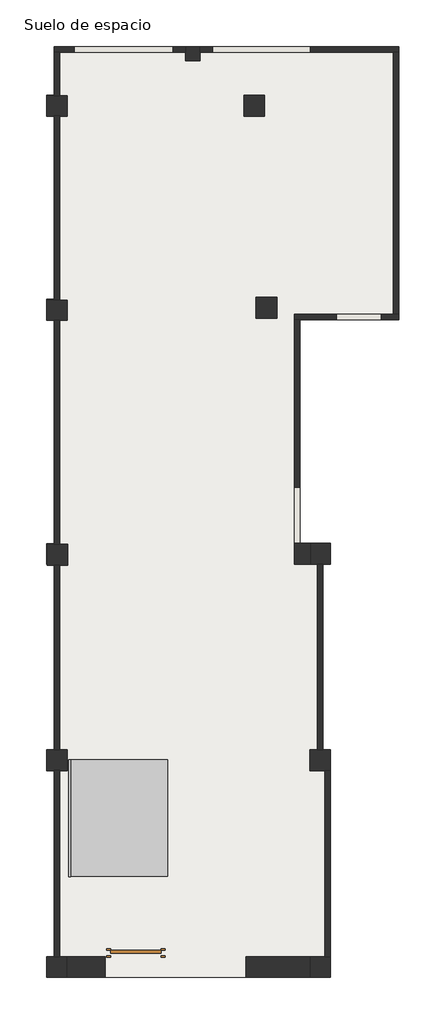
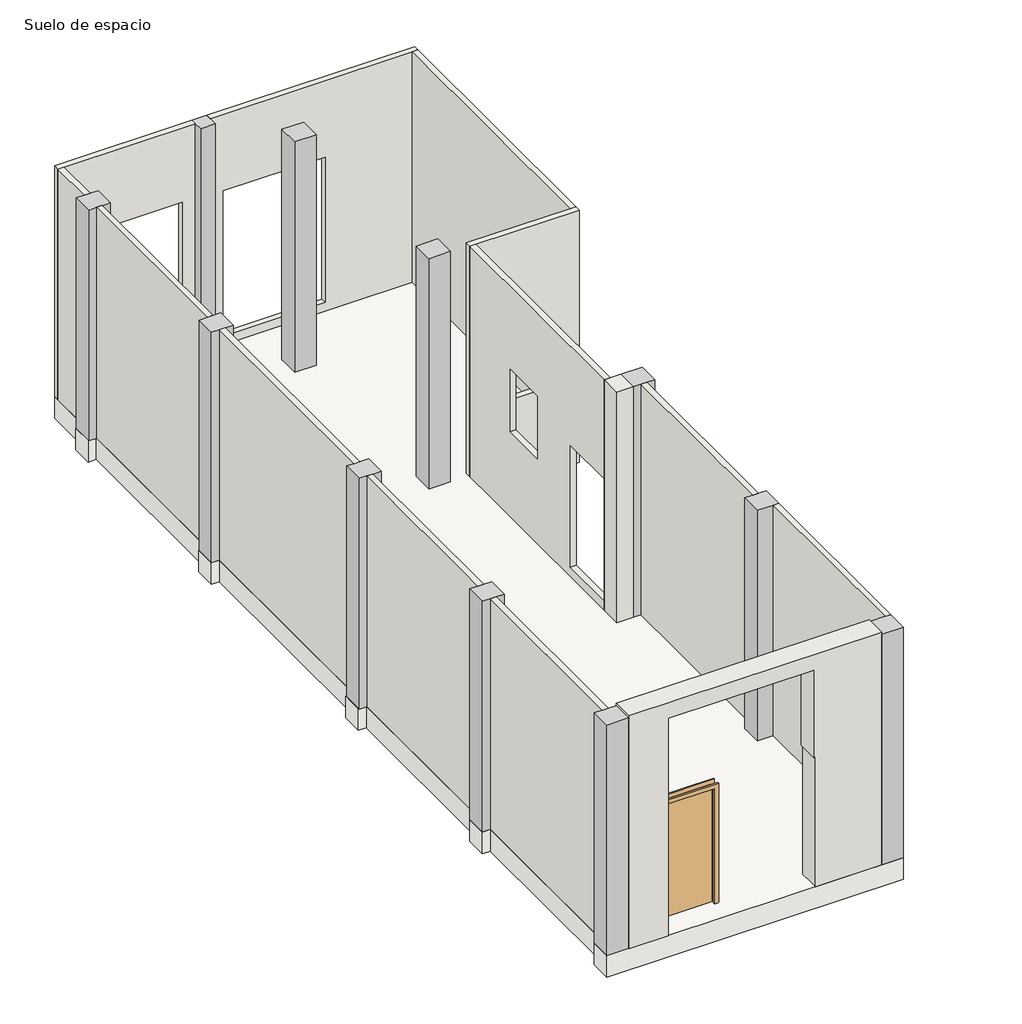
# One storey: 14 walls, 11 columns, 1 door, 1 railing, 1 ramp, 1 slab.
"""IFC4 building model written with IfcOpenShell, lengths in millimetres."""

import ifcopenshell
import ifcopenshell.guid

model = None  # the IFC model being written
_history = None  # IfcOwnerHistory: only IFC2X3 demands one
_inside = {}  # id of a spatial element -> (the spatial element, [elements in it])
_under = {}  # id of a project, library or spatial element -> (it, [spatial elements below it])
_declared = {}  # id of a project -> (the project, [libraries it declares])
_typed = {}  # id of a type object -> (the type object, [elements of that type])
_made_of = {}  # id of a material, layer set ... -> (it, [elements and type objects made of it])


def new_model(schema):
    """Start an empty IFC model of exactly this schema.

    Asked for "IFC4X3", IfcOpenShell would pick the latest addendum, in which some entities
    have other attributes; the version numbers below select the first issue.
    IFC2X3 requires an IfcOwnerHistory on every rooted entity: one is made here for all.
    """
    global model, _history
    if schema == "IFC4X3":
        model = ifcopenshell.file(schema_version=(4, 3, 0, 0))
    else:
        model = ifcopenshell.file(schema=schema)
    _inside.clear()
    _under.clear()
    _declared.clear()
    _typed.clear()
    _made_of.clear()
    _history = None
    if model.schema == "IFC2X3":
        org = make("IfcOrganization", Name="unknown")
        user = make(
            "IfcPersonAndOrganization",
            ThePerson=make("IfcPerson", FamilyName="unknown"),
            TheOrganization=org,
        )
        app = make(
            "IfcApplication",
            ApplicationDeveloper=org,
            Version="unknown",
            ApplicationFullName="unknown",
            ApplicationIdentifier="unknown",
        )
        _history = make(
            "IfcOwnerHistory",
            OwningUser=user,
            OwningApplication=app,
            ChangeAction="ADDED",
            CreationDate=0,
        )
    return model


def make(cls, **values):
    """One entity of the class cls with the attributes given. An attribute that is None is left unset."""
    return model.create_entity(
        cls, **{name: value for name, value in values.items() if value is not None}
    )


def rooted(cls, **values):
    """An entity with a GlobalId (a new one), such as an element, a storey or a relation."""
    return make(cls, GlobalId=ifcopenshell.guid.new(), OwnerHistory=_history, **values)


def si_unit(unit_type, name, prefix=None):
    """IfcSIUnit, for example si_unit("LENGTHUNIT", "METRE", prefix="MILLI")."""
    return make("IfcSIUnit", UnitType=unit_type, Prefix=prefix, Name=name)


def assignment(units):
    """IfcUnitAssignment: the units of a project."""
    return None if units is None else make("IfcUnitAssignment", Units=units)


def point(xyz):
    """IfcCartesianPoint."""
    return None if xyz is None else make("IfcCartesianPoint", Coordinates=xyz)


def direction(xyz):
    """IfcDirection."""
    return None if xyz is None else make("IfcDirection", DirectionRatios=xyz)


def frame(location, z_axis=None, x_axis=None):
    """IfcAxis2Placement3D, a coordinate frame: its origin and axes. An axis left out is left unset."""
    return make(
        "IfcAxis2Placement3D",
        Location=point(location),
        Axis=direction(z_axis),
        RefDirection=direction(x_axis),
    )


def origin():
    """The frame at (0, 0, 0) with its axes left unset."""
    return frame((0.0, 0.0, 0.0))


def origin_with_axes():
    """The frame at (0, 0, 0) with the z axis (0, 0, 1) and the x axis (1, 0, 0) written out."""
    return frame((0.0, 0.0, 0.0), z_axis=(0.0, 0.0, 1.0), x_axis=(1.0, 0.0, 0.0))


def place(relative_to, where):
    """IfcLocalPlacement: puts the frame where relative to a parent placement (None: the world)."""
    return make(
        "IfcLocalPlacement", PlacementRelTo=relative_to, RelativePlacement=where
    )


def context(
    kind, dimensions, precision=None, world=None, true_north=None, identifier=None
):
    """IfcGeometricRepresentationContext, for example the 3D "Model" context."""
    return make(
        "IfcGeometricRepresentationContext",
        ContextIdentifier=identifier,
        ContextType=kind,
        CoordinateSpaceDimension=dimensions,
        Precision=precision,
        WorldCoordinateSystem=world,
        TrueNorth=true_north,
    )


def project(units=None, contexts=None):
    """IfcProject with its units and contexts."""
    return rooted(
        "IfcProject",
        Name="project",
        RepresentationContexts=contexts,
        UnitsInContext=assignment(units),
    )


def spatial(cls, under=None, at=None, **own):
    """A site, building, storey or space (cls), placed at a placement, below another one or the project."""
    s = rooted(cls, ObjectPlacement=at, **own)
    if under is not None:
        _under.setdefault(under.id(), (under, []))[1].append(s)
    return s


def polyline(points):
    """IfcPolyline through the points."""
    return make("IfcPolyline", Points=[point(p) for p in points])


def ellipse_curve(where, semi_axis1, semi_axis2):
    """IfcEllipse in the frame where."""
    return make(
        "IfcEllipse", Position=where, SemiAxis1=semi_axis1, SemiAxis2=semi_axis2
    )


def outline(outer, holes=None, kind="AREA"):
    """IfcArbitraryClosedProfileDef: a profile drawn as a closed curve; with holes, ...WithVoids."""
    if holes is None:
        return make("IfcArbitraryClosedProfileDef", ProfileType=kind, OuterCurve=outer)
    return make(
        "IfcArbitraryProfileDefWithVoids",
        ProfileType=kind,
        OuterCurve=outer,
        InnerCurves=holes,
    )


def extrude(swept, where, along, depth):
    """IfcExtrudedAreaSolid: the profile swept, set in the frame where, extruded along a direction by depth."""
    return make(
        "IfcExtrudedAreaSolid",
        SweptArea=swept,
        Position=where,
        ExtrudedDirection=direction(along),
        Depth=depth,
    )


def faces_of(points, faces, orient=None, outer=None):
    """IfcFace entities. A face is a list of loops; a loop is a list of indices into points, from 0.

    orient and outer hold one flag for each loop. By default every Orientation is true, the
    first loop of a face is its IfcFaceOuterBound and the others are IfcFaceBound.
    """
    made = []
    for i, loops in enumerate(faces):
        bounds = []
        for j, loop in enumerate(loops):
            is_outer = j == 0 if outer is None else outer[i][j]
            bounds.append(
                make(
                    "IfcFaceOuterBound" if is_outer else "IfcFaceBound",
                    Bound=make("IfcPolyLoop", Polygon=[points[k] for k in loop]),
                    Orientation=True if orient is None else orient[i][j],
                )
            )
        made.append(make("IfcFace", Bounds=bounds))
    return made


def faceted_brep(points, faces, orient=None, outer=None, voids=None):
    """IfcFacetedBrep: a solid bounded by flat faces; with voids (closed shells), ...WithVoids."""
    shared = [point(p) for p in points]
    hull = make("IfcClosedShell", CfsFaces=faces_of(shared, faces, orient, outer))
    if voids is None:
        return make("IfcFacetedBrep", Outer=hull)
    return make(
        "IfcFacetedBrepWithVoids",
        Outer=hull,
        Voids=[
            make(cls, CfsFaces=faces_of(shared, fs, o, b)) for cls, fs, o, b in voids
        ],
    )


def shape(context_of_items, identifier, shape_type, items):
    """IfcShapeRepresentation: the items that make up one representation, for example the "Body"."""
    return make(
        "IfcShapeRepresentation",
        ContextOfItems=context_of_items,
        RepresentationIdentifier=identifier,
        RepresentationType=shape_type,
        Items=items,
    )


def source(mapping_origin, context_of_items, identifier, shape_type, items):
    """IfcRepresentationMap: a shape defined once, which mapped items show again and again."""
    return make(
        "IfcRepresentationMap",
        MappingOrigin=mapping_origin,
        MappedRepresentation=shape(context_of_items, identifier, shape_type, items),
    )


def transform(
    local_origin,
    x_axis=None,
    y_axis=None,
    z_axis=None,
    scale=None,
    scale2=None,
    scale3=None,
    uniform=True,
):
    """IfcCartesianTransformationOperator3D, or its non-uniform kind. x_axis, y_axis, z_axis: its Axis1, 2, 3."""
    if uniform:
        return make(
            "IfcCartesianTransformationOperator3D",
            Axis1=direction(x_axis),
            Axis2=direction(y_axis),
            LocalOrigin=point(local_origin),
            Scale=scale,
            Axis3=direction(z_axis),
        )
    return make(
        "IfcCartesianTransformationOperator3DnonUniform",
        Axis1=direction(x_axis),
        Axis2=direction(y_axis),
        LocalOrigin=point(local_origin),
        Scale=scale,
        Axis3=direction(z_axis),
        Scale2=scale2,
        Scale3=scale3,
    )


def mapped(mapping_source, mapping_target):
    """IfcMappedItem: shows the shape of a source again, moved by a transform."""
    return make(
        "IfcMappedItem", MappingSource=mapping_source, MappingTarget=mapping_target
    )


def made_of(thing, what):
    """Note that an element or type object is made of a material, layer set ...; save() writes the relation."""
    if what is not None:
        _made_of.setdefault(what.id(), (what, []))[1].append(thing)
    return thing


def element(
    cls,
    number,
    at=None,
    inside=None,
    cuts=None,
    type_object=None,
    material=None,
    context=None,
    identifier="Body",
    shape_type=None,
    held_by="IfcProductDefinitionShape",
    body=None,
    shapes=None,
    **own,
):
    """One element of the class cls, such as IfcWall. Its Tag is "e" and its number.

    at: its placement. inside: the storey or other place that contains it. cuts: it is an
    opening in that element (IfcRelVoidsElement). A single representation is given by context,
    identifier, shape_type and body (its items); several are given by shapes. held_by: the class
    of the entity that holds the representations. save() writes the other relations.
    """
    e = rooted(cls, Tag="e%d" % number, ObjectPlacement=at, **own)
    if body is not None:
        shapes = [shape(context, identifier, shape_type, body)]
    if shapes is not None:
        e.Representation = make(held_by, Representations=shapes)
    if inside is not None:
        _inside.setdefault(inside.id(), (inside, []))[1].append(e)
    if cuts is not None:
        rooted(
            "IfcRelVoidsElement", RelatingBuildingElement=cuts, RelatedOpeningElement=e
        )
    if type_object is not None:
        _typed.setdefault(type_object.id(), (type_object, []))[1].append(e)
    return made_of(e, material)


def aggregate(whole, parts):
    """IfcRelAggregates: a whole, such as a stair, and the parts it consists of."""
    return rooted("IfcRelAggregates", RelatingObject=whole, RelatedObjects=parts)


def save(model, path):
    """Write the relations noted so far, then the file.

    IfcRelAggregates (storeys below a building ...), IfcRelContainedInSpatialStructure (elements
    in a storey), IfcRelDefinesByType, IfcRelAssociatesMaterial and IfcRelDeclares: one each for
    every whole, place, type object, material and project.
    """
    for whole, parts in _under.values():
        aggregate(whole, parts)
    for where, things in _inside.values():
        rooted(
            "IfcRelContainedInSpatialStructure",
            RelatedElements=things,
            RelatingStructure=where,
        )
    for kind, things in _typed.values():
        rooted("IfcRelDefinesByType", RelatedObjects=things, RelatingType=kind)
    for what, things in _made_of.values():
        rooted("IfcRelAssociatesMaterial", RelatedObjects=things, RelatingMaterial=what)
    for by, libraries in _declared.values():
        rooted("IfcRelDeclares", RelatingContext=by, RelatedDefinitions=libraries)
    model.write(path)


def plane_surface(at):
    """IfcPlane: the flat surface through the origin of the frame at, square to its z axis."""
    return make("IfcPlane", Position=at)


def cylinder_surface(at, radius):
    """IfcCylindricalSurface: all points at the distance radius from the z axis of the frame at."""
    return make("IfcCylindricalSurface", Position=at, Radius=radius)


def advanced_brep(points, edges, surfaces, faces):
    """IfcAdvancedBrep: a solid bounded by faces that lie on surfaces and meet in shared edges.

    An edge is (start, end): straight between two places in points (the first is 0);
    or (start, end, curve); or (start, end, curve, False) where it runs against its curve.
    A face is (place in surfaces, loops), or (place, loops, False) where it looks against
    its surface's normal. A loop lists edges by number (the first is 1), with a minus sign
    where the edge is run from its end to its start. The first loop is the outer one.
    """
    corners = [point(p) for p in points]
    vertices = [make("IfcVertexPoint", VertexGeometry=c) for c in corners]
    made = []
    for start, end, *more in edges:
        made.append(
            make(
                "IfcEdgeCurve",
                EdgeStart=vertices[start],
                EdgeEnd=vertices[end],
                EdgeGeometry=more[0] if more else make("IfcPolyline", Points=[corners[start], corners[end]]),
                SameSense=more[1] if len(more) > 1 else True,
            )
        )
    hull = []
    for where, loops, *sense in faces:
        bounds = []
        for j, loop in enumerate(loops):
            ring = [make("IfcOrientedEdge", EdgeElement=made[abs(k) - 1], Orientation=k > 0) for k in loop]
            bounds.append(
                make(
                    "IfcFaceOuterBound" if j == 0 else "IfcFaceBound",
                    Bound=make("IfcEdgeLoop", EdgeList=ring),
                    Orientation=True,
                )
            )
        hull.append(make("IfcAdvancedFace", Bounds=bounds, FaceSurface=surfaces[where], SameSense=sense[0] if sense else True))
    return make("IfcAdvancedBrep", Outer=make("IfcClosedShell", CfsFaces=hull))


def m_rectangular_column_380_x_380mm_f7aa0fc7(model_context):
    return source(origin(), model_context, "Body", "SweptSolid", [
        extrude(outline(polyline([(190.0, 190.0), (190.0, -190.0), (-190.0, -190.0), (-190.0, 190.0), (190.0, 190.0)])), frame((0.0, 0.0, 40.0), z_axis=(0.0, 0.0, 1.0), x_axis=(1.0, 0.0, 0.0)), (0.0, 0.0, 1.0), 4260.0),
    ])


def m_single_flush_0915_x_2134mm_17617764(model_context):
    return source(origin(), model_context, "Body", "SweptSolid", [
        extrude(outline(polyline([(2210.0, -533.5), (0.0, -533.5), (0.0, -457.5), (2134.0, -457.5), (2134.0, 457.5), (0.0, 457.5), (0.0, 533.5), (2210.0, 533.5), (2210.0, -533.5)])), frame((0.0, -75.0, 0.0), z_axis=(0.0, 1.0, 0.0), x_axis=(0.0, 0.0, 1.0)), (0.0, 0.0, 1.0), 25.0),
        extrude(outline(polyline([(2210.0, 533.5), (2210.0, -533.5), (0.0, -533.5), (0.0, -457.5), (2134.0, -457.5), (2134.0, 457.5), (0.0, 457.5), (0.0, 533.5), (2210.0, 533.5)])), frame((0.0, 50.0, 0.0), z_axis=(0.0, 1.0, 0.0), x_axis=(0.0, 0.0, 1.0)), (0.0, 0.0, 1.0), 25.0),
        extrude(outline(polyline([(457.5, 1.0), (457.5, -50.0), (-457.5, -50.0), (-457.5, 1.0), (457.5, 1.0)])), origin_with_axes(), (0.0, 0.0, 1.0), 2134.0),
    ])


def ramp_1_66d68c1d(model_context):
    return source(origin(), model_context, "Body", "SweptSolid", [
        extrude(outline(polyline([(-178.9025016, 40.0), (1960.7723822, 200.0), (1960.7723822, 49.5812066), (-178.9025016, -110.4187934), (-178.9025016, 40.0)])), frame((5764.7203549, 0.0, 0.0), z_axis=(1.0, 0.0, 0.0), x_axis=(0.0, 1.0, 0.0)), (0.0, 0.0, 1.0), 1790.0),
    ])


model = new_model("IFC4")

# Units and contexts
model_context = context("Model", 3, world=origin())
ifc_project = project(units=[si_unit("LENGTHUNIT", "METRE", prefix="MILLI")], contexts=[model_context])

# Site, building, storey
site = spatial("IfcSite", under=ifc_project)
building = spatial("IfcBuilding", under=site)
storey = spatial("IfcBuildingStorey", under=building, Name="Suelo de espacio", Elevation=40.0)

# Columns
placement = place(None, origin())
element("IfcColumn", 1, ObjectType="M_Rectangular Column : 260 x 260mm", at=placement, inside=storey, context=model_context, shape_type="Brep", body=[
    faceted_brep([(8142.3508412, 14950.939444, 4300.0), (7882.3508412, 14950.939444, 4300.0), (7882.3508412, 14850.939444, 4300.0), (7882.3508412, 14690.939444, 4300.0), (8142.3508412, 14690.939444, 4300.0), (8142.3508412, 14850.939444, 4300.0), (8142.3508412, 14950.939444, 40.0), (8142.3508412, 14850.939444, 40.0), (8142.3508412, 14690.939444, 40.0), (7882.3508412, 14690.939444, 40.0), (7882.3508412, 14850.939444, 40.0), (7882.3508412, 14950.939444, 40.0)], [[[0, 1, 2, 3, 4, 5]], [[6, 7, 8, 9, 10, 11]], [[1, 0, 6, 11]], [[3, 2, 1, 11, 10, 9]], [[4, 3, 9, 8]], [[0, 5, 4, 8, 7, 6]]]),
])
element("IfcColumn", 2, ObjectType="M_Rectangular Column : 380 x 370mm", at=placement, inside=storey, context=model_context, shape_type="Brep", body=[
    faceted_brep([(5722.3508412, 10330.939444, 4300.0), (5342.3508412, 10330.939444, 4300.0), (5342.3508412, 9960.939444, 4300.0), (5482.3508412, 9960.939444, 4300.0), (5582.3508412, 9960.939444, 4300.0), (5722.3508412, 9960.939444, 4300.0), (5722.3508412, 10330.939444, 40.0), (5722.3508412, 9960.939444, 40.0), (5582.3508412, 9960.939444, 40.0), (5482.3508412, 9960.939444, 40.0), (5342.3508412, 9960.939444, 40.0), (5342.3508412, 10330.939444, 40.0)], [[[0, 1, 2, 3, 4, 5]], [[6, 7, 8, 9, 10, 11]], [[1, 0, 6, 11]], [[2, 1, 11, 10]], [[5, 4, 3, 2, 10, 9, 8, 7]], [[0, 5, 7, 6]]]),
])
element("IfcColumn", 3, ObjectType="M_Rectangular Column : 380 x 370mm", at=placement, inside=storey, context=model_context, shape_type="Brep", body=[
    faceted_brep([(5722.3508412, 14050.939444, 4300.0), (5582.3508412, 14050.939444, 4300.0), (5482.3508412, 14050.939444, 4300.0), (5342.3508412, 14050.939444, 4300.0), (5342.3508412, 13680.939444, 4300.0), (5482.3508412, 13680.939444, 4300.0), (5482.3508412, 13685.939444, 4300.0), (5582.3508412, 13685.939444, 4300.0), (5582.3508412, 13680.939444, 4300.0), (5722.3508412, 13680.939444, 4300.0), (5722.3508412, 14050.939444, 40.0), (5722.3508412, 13680.939444, 40.0), (5582.3508412, 13680.939444, 40.0), (5582.3508412, 13685.939444, 40.0), (5482.3508412, 13685.939444, 40.0), (5482.3508412, 13680.939444, 40.0), (5342.3508412, 13680.939444, 40.0), (5342.3508412, 14050.939444, 40.0), (5482.3508412, 14050.939444, 40.0), (5582.3508412, 14050.939444, 40.0)], [[[0, 1, 2, 3, 4, 5, 6, 7, 8, 9]], [[10, 11, 12, 13, 14, 15, 16, 17, 18, 19]], [[3, 2, 1, 0, 10, 19, 18, 17]], [[4, 3, 17, 16]], [[4, 16, 15, 5]], [[0, 9, 11, 10]], [[7, 13, 12, 8]], [[14, 6, 5, 15]], [[13, 7, 6, 14]], [[11, 9, 8, 12]]]),
])
element("IfcColumn", 4, ObjectType="M_Rectangular Column : 380 x 380mm", at=placement, inside=storey, context=model_context, shape_type="Brep", body=[
    faceted_brep([(5722.3508412, -1629.060556, 4300.0), (5582.3508412, -1629.060556, 4300.0), (5482.3508412, -1629.060556, 4300.0), (5342.3508412, -1629.060556, 4300.0), (5342.3508412, -2009.060556, 4300.0), (5722.3508412, -2009.060556, 4300.0), (5722.3508412, -1629.060556, 40.0), (5722.3508412, -2009.060556, 40.0), (5342.3508412, -2009.060556, 40.0), (5342.3508412, -1629.060556, 40.0), (5482.3508412, -1629.060556, 40.0), (5582.3508412, -1629.060556, 40.0)], [[[0, 1, 2, 3, 4, 5]], [[6, 7, 8, 9, 10, 11]], [[3, 2, 1, 0, 6, 11, 10, 9]], [[4, 3, 9, 8]], [[5, 4, 8, 7]], [[0, 5, 7, 6]]]),
])
element("IfcColumn", 5, ObjectType="M_Rectangular Column : 380 x 380mm", at=placement, inside=storey, context=model_context, shape_type="Brep", body=[
    faceted_brep([(10522.3508412, -1629.060556, 4300.0), (10422.3508412, -1629.060556, 4300.0), (10142.3508412, -1629.060556, 4300.0), (10142.3508412, -2009.060556, 4300.0), (10522.3508412, -2009.060556, 4300.0), (10522.3508412, -1629.060556, 40.0), (10522.3508412, -2009.060556, 40.0), (10142.3508412, -2009.060556, 40.0), (10142.3508412, -1629.060556, 40.0), (10422.3508412, -1629.060556, 40.0)], [[[0, 1, 2, 3, 4]], [[5, 6, 7, 8, 9]], [[2, 1, 0, 5, 9, 8]], [[3, 2, 8, 7]], [[4, 3, 7, 6]], [[0, 4, 6, 5]]]),
])
element("IfcColumn", 6, ObjectType="M_Rectangular Column : 380 x 380mm", at=placement, inside=storey, context=model_context, shape_type="Brep", body=[
    faceted_brep([(5722.3508412, 2140.939444, 4300.0), (5582.3508412, 2140.939444, 4300.0), (5482.3508412, 2140.939444, 4300.0), (5342.3508412, 2140.939444, 4300.0), (5342.3508412, 1760.939444, 4300.0), (5482.3508412, 1760.939444, 4300.0), (5482.3508412, 1761.3849652, 4300.0), (5582.3508412, 1761.3849652, 4300.0), (5582.3508412, 1760.939444, 4300.0), (5722.3508412, 1760.939444, 4300.0), (5722.3508412, 2140.939444, 40.0), (5722.3508412, 1760.939444, 40.0), (5582.3508412, 1760.939444, 40.0), (5582.3508412, 1761.3849652, 40.0), (5482.3508412, 1761.3849652, 40.0), (5482.3508412, 1760.939444, 40.0), (5342.3508412, 1760.939444, 40.0), (5342.3508412, 2140.939444, 40.0), (5482.3508412, 2140.939444, 40.0), (5582.3508412, 2140.939444, 40.0)], [[[0, 1, 2, 3, 4, 5, 6, 7, 8, 9]], [[10, 11, 12, 13, 14, 15, 16, 17, 18, 19]], [[3, 2, 1, 0, 10, 19, 18, 17]], [[4, 3, 17, 16]], [[4, 16, 15, 5]], [[0, 9, 11, 10]], [[7, 13, 12, 8]], [[14, 6, 5, 15]], [[11, 9, 8, 12]], [[13, 7, 6, 14]]]),
])
element("IfcColumn", 7, ObjectType="M_Rectangular Column : 380 x 380mm", at=placement, inside=storey, context=model_context, shape_type="Brep", body=[
    faceted_brep([(10522.3508412, 2140.939444, 4300.0), (10382.3508412, 2140.939444, 4300.0), (10282.3508412, 2140.939444, 4300.0), (10142.3508412, 2140.939444, 4300.0), (10142.3508412, 1760.939444, 4300.0), (10422.3508412, 1760.939444, 4300.0), (10522.3508412, 1760.939444, 4300.0), (10522.3508412, 2140.939444, 40.0), (10522.3508412, 1760.939444, 40.0), (10422.3508412, 1760.939444, 40.0), (10142.3508412, 1760.939444, 40.0), (10142.3508412, 2140.939444, 40.0), (10282.3508412, 2140.939444, 40.0), (10382.3508412, 2140.939444, 40.0)], [[[0, 1, 2, 3, 4, 5, 6]], [[7, 8, 9, 10, 11, 12, 13]], [[3, 2, 1, 0, 7, 13, 12, 11]], [[4, 3, 11, 10]], [[6, 5, 4, 10, 9, 8]], [[0, 6, 8, 7]]]),
])
element("IfcColumn", 8, ObjectType="M_Rectangular Column : 380 x 380mm", at=placement, inside=storey, context=model_context, shape_type="Brep", body=[
    faceted_brep([(5732.3508412, 5880.939444, 4300.0), (5582.3508412, 5880.939444, 4300.0), (5482.3508412, 5880.939444, 4300.0), (5352.3508412, 5880.939444, 4300.0), (5352.3508412, 5500.939444, 4300.0), (5482.3508412, 5500.939444, 4300.0), (5582.3508412, 5500.939444, 4300.0), (5732.3508412, 5500.939444, 4300.0), (5732.3508412, 5880.939444, 40.0), (5732.3508412, 5500.939444, 40.0), (5582.3508412, 5500.939444, 40.0), (5482.3508412, 5500.939444, 40.0), (5352.3508412, 5500.939444, 40.0), (5352.3508412, 5880.939444, 40.0), (5482.3508412, 5880.939444, 40.0), (5582.3508412, 5880.939444, 40.0)], [[[0, 1, 2, 3, 4, 5, 6, 7]], [[8, 9, 10, 11, 12, 13, 14, 15]], [[3, 2, 1, 0, 8, 15, 14, 13]], [[4, 3, 13, 12]], [[7, 6, 5, 4, 12, 11, 10, 9]], [[0, 7, 9, 8]]]),
])
element("IfcColumn", 9, ObjectType="M_Rectangular Column : 380 x 380mm", at=placement, inside=storey, context=model_context, shape_type="Brep", body=[
    faceted_brep([(10522.3508412, 5520.939444, 4300.0), (10522.3508412, 5900.939444, 4300.0), (10152.3508412, 5900.939444, 4300.0), (10152.3508412, 5520.939444, 4300.0), (10282.3508412, 5520.939444, 4300.0), (10382.3508412, 5520.939444, 4300.0), (10522.3508412, 5900.939444, 40.0), (10522.3508412, 5520.939444, 40.0), (10382.3508412, 5520.939444, 40.0), (10282.3508412, 5520.939444, 40.0), (10152.3508412, 5520.939444, 40.0), (10152.3508412, 5900.939444, 40.0)], [[[0, 1, 2, 3, 4, 5]], [[6, 7, 8, 9, 10, 11]], [[1, 6, 11, 2]], [[7, 0, 5, 4, 3, 10, 9, 8]], [[1, 0, 7, 6]], [[3, 2, 11, 10]]]),
])
m_rectangular_column_380_x_380mm_shape = m_rectangular_column_380_x_380mm_f7aa0fc7(model_context)
element("IfcColumn", 10, ObjectType="M_Rectangular Column : 380 x 380mm", at=placement, inside=storey, context=model_context, shape_type="MappedRepresentation", body=[
    mapped(m_rectangular_column_380_x_380mm_shape, transform((9132.3508412, 13870.939444, 0.0), x_axis=(1.0, 0.0, 0.0), y_axis=(0.0, 1.0, 0.0), z_axis=(0.0, 0.0, 1.0))),
])
element("IfcColumn", 11, ObjectType="M_Rectangular Column : 380 x 380mm", at=placement, inside=storey, context=model_context, shape_type="MappedRepresentation", body=[
    mapped(m_rectangular_column_380_x_380mm_shape, transform((9352.3508412, 10190.939444, 0.0), x_axis=(1.0, 0.0, 0.0), y_axis=(0.0, 1.0, 0.0), z_axis=(0.0, 0.0, 1.0))),
])

# Door
m_single_flush_0915_x_2134mm_shape = m_single_flush_0915_x_2134mm_17617764(model_context)
element("IfcDoor", 12, ObjectType="M_Single-Flush : 0915 x 2134mm", at=placement, inside=storey, context=model_context, shape_type="MappedRepresentation", body=[
    mapped(m_single_flush_0915_x_2134mm_shape, transform((6972.3508412, -1564.060556, 40.0), x_axis=(-1.0, 0.0, 0.0), y_axis=(0.0, -1.0, 0.0), z_axis=(0.0, 0.0, 1.0))),
])

# Railing
element("IfcRailing", 13, ObjectType="900mm Pipe", at=placement, inside=storey, context=model_context, shape_type="AdvancedBrep", body=[
    advanced_brep(
    [(5784.7203549, -178.9025016, 919.9441609), (5744.7203549, -178.9025016, 919.9441609), (5784.7203549, 1960.7723822, 1079.9441609), (5744.7203549, 1960.7723822, 1079.9441609)],
    [
        (0, 1, ellipse_curve(frame((5764.7203549, -178.9025016, 919.9441609), z_axis=(0.0, -1.0, 0.0), x_axis=(0.0, 0.0, -0.9999999999999999)), 20.0558391, 20.0)),
        (1, 0, ellipse_curve(frame((5764.7203549, -178.9025016, 919.9441609), z_axis=(0.0, -1.0, 0.0), x_axis=(0.0, 0.0, -0.9999999999999999)), 20.0558391, 20.0)),
        (2, 3, ellipse_curve(frame((5764.7203549, 1960.7723822, 1079.9441609), z_axis=(0.0, 1.0, 0.0), x_axis=(0.0, 0.0, -0.9999999999999999)), 20.0558391, 20.0)),
        (3, 2, ellipse_curve(frame((5764.7203549, 1960.7723822, 1079.9441609), z_axis=(0.0, 1.0, 0.0), x_axis=(0.0, 0.0, -0.9999999999999999)), 20.0558391, 20.0)),
        (0, 2),
        (3, 1),
    ],
    [
        plane_surface(frame((5764.7203549, -178.9025016, 940.0), z_axis=(0.0, -1.0, 0.0), x_axis=(0.0, 0.0, 1.0))),
        plane_surface(frame((5764.7203549, 1960.7723822, 1100.0), z_axis=(0.0, 1.0, 0.0), x_axis=(0.0, 0.0, 1.0))),
        cylinder_surface(frame((5764.7203549, -177.4111112, 920.0556837), z_axis=(0.0, -0.9972158174462339, -0.07456952081809042), x_axis=(-1.0, 0.0, 0.0)), 20.0),
    ],
    [
        (0, [[1, 2]]),
        (1, [[3, 4]]),
        (2, [[-1, 5, -4, 6]]),
        (2, [[-2, -6, -3, -5]]),
    ],
),
    advanced_brep(
    [(5749.7203549, -178.9025016, 799.9581207), (5779.7203549, -178.9025016, 799.9581207), (5749.7203549, 1960.7723822, 959.9581207), (5779.7203549, 1960.7723822, 959.9581207)],
    [
        (0, 1, ellipse_curve(frame((5764.7203549, -178.9025016, 799.9581207), z_axis=(0.0, -1.0, 0.0), x_axis=(0.0, 0.0, -0.9999999999999999)), 15.0418793, 15.0)),
        (1, 0, ellipse_curve(frame((5764.7203549, -178.9025016, 799.9581207), z_axis=(0.0, -1.0, 0.0), x_axis=(0.0, 0.0, -0.9999999999999999)), 15.0418793, 15.0)),
        (2, 3, ellipse_curve(frame((5764.7203549, 1960.7723822, 959.9581207), z_axis=(0.0, 1.0, 0.0), x_axis=(0.0, 0.0, -0.9999999999999999)), 15.0418793, 15.0)),
        (3, 2, ellipse_curve(frame((5764.7203549, 1960.7723822, 959.9581207), z_axis=(0.0, 1.0, 0.0), x_axis=(0.0, 0.0, -0.9999999999999999)), 15.0418793, 15.0)),
        (0, 2),
        (3, 1),
    ],
    [
        plane_surface(frame((5764.7203549, -178.9025016, 815.0), z_axis=(0.0, -1.0, 0.0), x_axis=(0.0, 0.0, 1.0))),
        plane_surface(frame((5764.7203549, 1960.7723822, 975.0), z_axis=(0.0, 1.0, 0.0), x_axis=(0.0, 0.0, 1.0))),
        cylinder_surface(frame((5764.7203549, -177.7839588, 800.0417627), z_axis=(0.0, -0.9972158174462339, -0.07456952081809042), x_axis=(1.0, 0.0, 0.0)), 15.0),
    ],
    [
        (0, [[1, 2]]),
        (1, [[3, 4]]),
        (2, [[-1, 5, -4, 6]]),
        (2, [[-2, -6, -3, -5]]),
    ],
),
    advanced_brep(
    [(5749.7203549, -178.9025016, 674.9581207), (5779.7203549, -178.9025016, 674.9581207), (5749.7203549, 1960.7723822, 834.9581207), (5779.7203549, 1960.7723822, 834.9581207)],
    [
        (0, 1, ellipse_curve(frame((5764.7203549, -178.9025016, 674.9581207), z_axis=(0.0, -1.0, 0.0), x_axis=(0.0, 0.0, -0.9999999999999999)), 15.0418793, 15.0)),
        (1, 0, ellipse_curve(frame((5764.7203549, -178.9025016, 674.9581207), z_axis=(0.0, -1.0, 0.0), x_axis=(0.0, 0.0, -0.9999999999999999)), 15.0418793, 15.0)),
        (2, 3, ellipse_curve(frame((5764.7203549, 1960.7723822, 834.9581207), z_axis=(0.0, 1.0, 0.0), x_axis=(0.0, 0.0, -0.9999999999999999)), 15.0418793, 15.0)),
        (3, 2, ellipse_curve(frame((5764.7203549, 1960.7723822, 834.9581207), z_axis=(0.0, 1.0, 0.0), x_axis=(0.0, 0.0, -0.9999999999999999)), 15.0418793, 15.0)),
        (0, 2),
        (3, 1),
    ],
    [
        plane_surface(frame((5764.7203549, -178.9025016, 690.0), z_axis=(0.0, -1.0, 0.0), x_axis=(0.0, 0.0, 1.0))),
        plane_surface(frame((5764.7203549, 1960.7723822, 850.0), z_axis=(0.0, 1.0, 0.0), x_axis=(0.0, 0.0, 1.0))),
        cylinder_surface(frame((5764.7203549, -177.7839588, 675.0417627), z_axis=(0.0, -0.9972158174462339, -0.07456952081809042), x_axis=(1.0, 0.0, 0.0)), 15.0),
    ],
    [
        (0, [[1, 2]]),
        (1, [[3, 4]]),
        (2, [[-1, 5, -4, 6]]),
        (2, [[-2, -6, -3, -5]]),
    ],
),
    advanced_brep(
    [(5749.7203549, -178.9025016, 549.9581207), (5779.7203549, -178.9025016, 549.9581207), (5749.7203549, 1960.7723822, 709.9581207), (5779.7203549, 1960.7723822, 709.9581207)],
    [
        (0, 1, ellipse_curve(frame((5764.7203549, -178.9025016, 549.9581207), z_axis=(0.0, -1.0, 0.0), x_axis=(0.0, 0.0, -0.9999999999999999)), 15.0418793, 15.0)),
        (1, 0, ellipse_curve(frame((5764.7203549, -178.9025016, 549.9581207), z_axis=(0.0, -1.0, 0.0), x_axis=(0.0, 0.0, -0.9999999999999999)), 15.0418793, 15.0)),
        (2, 3, ellipse_curve(frame((5764.7203549, 1960.7723822, 709.9581207), z_axis=(0.0, 1.0, 0.0), x_axis=(0.0, 0.0, -0.9999999999999999)), 15.0418793, 15.0)),
        (3, 2, ellipse_curve(frame((5764.7203549, 1960.7723822, 709.9581207), z_axis=(0.0, 1.0, 0.0), x_axis=(0.0, 0.0, -0.9999999999999999)), 15.0418793, 15.0)),
        (0, 2),
        (3, 1),
    ],
    [
        plane_surface(frame((5764.7203549, -178.9025016, 565.0), z_axis=(0.0, -1.0, 0.0), x_axis=(0.0, 0.0, 1.0))),
        plane_surface(frame((5764.7203549, 1960.7723822, 725.0), z_axis=(0.0, 1.0, 0.0), x_axis=(0.0, 0.0, 1.0))),
        cylinder_surface(frame((5764.7203549, -177.7839588, 550.0417627), z_axis=(0.0, -0.9972158174462339, -0.07456952081809042), x_axis=(1.0, 0.0, 0.0)), 15.0),
    ],
    [
        (0, [[1, 2]]),
        (1, [[3, 4]]),
        (2, [[-1, 5, -4, 6]]),
        (2, [[-2, -6, -3, -5]]),
    ],
),
    advanced_brep(
    [(5749.7203549, -178.9025016, 424.9581207), (5779.7203549, -178.9025016, 424.9581207), (5749.7203549, 1960.7723822, 584.9581207), (5779.7203549, 1960.7723822, 584.9581207)],
    [
        (0, 1, ellipse_curve(frame((5764.7203549, -178.9025016, 424.9581207), z_axis=(0.0, -1.0, 0.0), x_axis=(0.0, 0.0, -0.9999999999999999)), 15.0418793, 15.0)),
        (1, 0, ellipse_curve(frame((5764.7203549, -178.9025016, 424.9581207), z_axis=(0.0, -1.0, 0.0), x_axis=(0.0, 0.0, -0.9999999999999999)), 15.0418793, 15.0)),
        (2, 3, ellipse_curve(frame((5764.7203549, 1960.7723822, 584.9581207), z_axis=(0.0, 1.0, 0.0), x_axis=(0.0, 0.0, -0.9999999999999999)), 15.0418793, 15.0)),
        (3, 2, ellipse_curve(frame((5764.7203549, 1960.7723822, 584.9581207), z_axis=(0.0, 1.0, 0.0), x_axis=(0.0, 0.0, -0.9999999999999999)), 15.0418793, 15.0)),
        (0, 2),
        (3, 1),
    ],
    [
        plane_surface(frame((5764.7203549, -178.9025016, 440.0), z_axis=(0.0, -1.0, 0.0), x_axis=(0.0, 0.0, 1.0))),
        plane_surface(frame((5764.7203549, 1960.7723822, 600.0), z_axis=(0.0, 1.0, 0.0), x_axis=(0.0, 0.0, 1.0))),
        cylinder_surface(frame((5764.7203549, -177.7839588, 425.0417627), z_axis=(0.0, -0.9972158174462339, -0.07456952081809042), x_axis=(1.0, 0.0, 0.0)), 15.0),
    ],
    [
        (0, [[1, 2]]),
        (1, [[3, 4]]),
        (2, [[-1, 5, -4, 6]]),
        (2, [[-2, -6, -3, -5]]),
    ],
),
    advanced_brep(
    [(5749.7203549, -178.9025016, 299.9581207), (5779.7203549, -178.9025016, 299.9581207), (5749.7203549, 1960.7723822, 459.9581207), (5779.7203549, 1960.7723822, 459.9581207)],
    [
        (0, 1, ellipse_curve(frame((5764.7203549, -178.9025016, 299.9581207), z_axis=(0.0, -1.0, 0.0), x_axis=(0.0, 0.0, -0.9999999999999999)), 15.0418793, 15.0)),
        (1, 0, ellipse_curve(frame((5764.7203549, -178.9025016, 299.9581207), z_axis=(0.0, -1.0, 0.0), x_axis=(0.0, 0.0, -0.9999999999999999)), 15.0418793, 15.0)),
        (2, 3, ellipse_curve(frame((5764.7203549, 1960.7723822, 459.9581207), z_axis=(0.0, 1.0, 0.0), x_axis=(0.0, 0.0, -0.9999999999999999)), 15.0418793, 15.0)),
        (3, 2, ellipse_curve(frame((5764.7203549, 1960.7723822, 459.9581207), z_axis=(0.0, 1.0, 0.0), x_axis=(0.0, 0.0, -0.9999999999999999)), 15.0418793, 15.0)),
        (0, 2),
        (3, 1),
    ],
    [
        plane_surface(frame((5764.7203549, -178.9025016, 315.0), z_axis=(0.0, -1.0, 0.0), x_axis=(0.0, 0.0, 1.0))),
        plane_surface(frame((5764.7203549, 1960.7723822, 475.0), z_axis=(0.0, 1.0, 0.0), x_axis=(0.0, 0.0, 1.0))),
        cylinder_surface(frame((5764.7203549, -177.7839588, 300.0417627), z_axis=(0.0, -0.9972158174462339, -0.07456952081809042), x_axis=(1.0, 0.0, 0.0)), 15.0),
    ],
    [
        (0, [[1, 2]]),
        (1, [[3, 4]]),
        (2, [[-1, 5, -4, 6]]),
        (2, [[-2, -6, -3, -5]]),
    ],
),
    advanced_brep(
    [(5749.7203549, -178.9025016, 174.9581207), (5779.7203549, -178.9025016, 174.9581207), (5749.7203549, 1960.7723822, 334.9581207), (5779.7203549, 1960.7723822, 334.9581207)],
    [
        (0, 1, ellipse_curve(frame((5764.7203549, -178.9025016, 174.9581207), z_axis=(0.0, -1.0, 0.0), x_axis=(0.0, 0.0, -1.0)), 15.0418793, 15.0)),
        (1, 0, ellipse_curve(frame((5764.7203549, -178.9025016, 174.9581207), z_axis=(0.0, -1.0, 0.0), x_axis=(0.0, 0.0, -1.0)), 15.0418793, 15.0)),
        (2, 3, ellipse_curve(frame((5764.7203549, 1960.7723822, 334.9581207), z_axis=(0.0, 1.0, 0.0), x_axis=(0.0, 0.0, -1.0)), 15.0418793, 15.0)),
        (3, 2, ellipse_curve(frame((5764.7203549, 1960.7723822, 334.9581207), z_axis=(0.0, 1.0, 0.0), x_axis=(0.0, 0.0, -1.0)), 15.0418793, 15.0)),
        (0, 2),
        (3, 1),
    ],
    [
        plane_surface(frame((5764.7203549, -178.9025016, 190.0), z_axis=(0.0, -1.0, 0.0), x_axis=(0.0, 0.0, 1.0))),
        plane_surface(frame((5764.7203549, 1960.7723822, 350.0), z_axis=(0.0, 1.0, 0.0), x_axis=(0.0, 0.0, 1.0))),
        cylinder_surface(frame((5764.7203549, -177.7839588, 175.0417627), z_axis=(0.0, -0.9972158174462339, -0.07456952081809039), x_axis=(1.0, 0.0, 0.0)), 15.0),
    ],
    [
        (0, [[1, 2]]),
        (1, [[3, 4]]),
        (2, [[-1, 5, -4, 6]]),
        (2, [[-2, -6, -3, -5]]),
    ],
),
    advanced_brep(
    [(5777.2203549, 1821.0974984, 1049.443753), (5777.2203549, 1821.0974984, 189.5554313), (5752.2203549, 1821.0974984, 189.5554313), (5752.2203549, 1821.0974984, 1049.443753)],
    [
        (0, 1),
        (1, 2, ellipse_curve(frame((5764.7203549, 1821.0974984, 189.5554313), z_axis=(0.0, -0.07456952081809026, 0.9972158174462339), x_axis=(0.0, 0.9972158174462339, 0.07456952081808967)), 12.5348994, 12.5)),
        (2, 3),
        (3, 0, ellipse_curve(frame((5764.7203549, 1821.0974984, 1049.443753), z_axis=(0.0, 0.07456952081809023, -0.9972158174462339), x_axis=(0.0, 0.9972158174462339, 0.0745695208180897)), 12.5348994, 12.5)),
        (0, 3, ellipse_curve(frame((5764.7203549, 1821.0974984, 1049.443753), z_axis=(0.0, 0.07456952081809023, -0.9972158174462339), x_axis=(0.0, 0.9972158174462339, 0.0745695208180897)), 12.5348994, 12.5)),
        (2, 1, ellipse_curve(frame((5764.7203549, 1821.0974984, 189.5554313), z_axis=(0.0, -0.07456952081809026, 0.9972158174462339), x_axis=(0.0, 0.9972158174462339, 0.07456952081808967)), 12.5348994, 12.5)),
    ],
    [
        cylinder_surface(frame((5764.7203549, 1821.0974984, 89.5554313), z_axis=(0.0, 0.0, 1.0), x_axis=(-1.0, 0.0, 0.0)), 12.5),
        plane_surface(frame((5739.7203549, 1846.0974984, 1051.3131959), z_axis=(0.0, -0.07456952081809023, 0.9972158174462339), x_axis=(1.0, 0.0, 0.0))),
        plane_surface(frame((5739.7203549, 1796.0974984, 187.6859884), z_axis=(0.0, 0.07456952081809026, -0.9972158174462339), x_axis=(1.0, 0.0, 0.0))),
    ],
    [
        (0, [[1, 2, 3, 4]]),
        (0, [[-1, 5, -3, 6]]),
        (1, [[-4, -5]]),
        (2, [[-2, -6]]),
    ],
),
    advanced_brep(
    [(5777.2203549, 821.0974984, 974.6660374), (5777.2203549, 821.0974984, 114.7777156), (5752.2203549, 821.0974984, 114.7777156), (5752.2203549, 821.0974984, 974.6660374)],
    [
        (0, 1),
        (1, 2, ellipse_curve(frame((5764.7203549, 821.0974984, 114.7777156), z_axis=(0.0, -0.07456952081809026, 0.9972158174462339), x_axis=(0.0, 0.9972158174462339, 0.07456952081808967)), 12.5348994, 12.5)),
        (2, 3),
        (3, 0, ellipse_curve(frame((5764.7203549, 821.0974984, 974.6660374), z_axis=(0.0, 0.07456952081809023, -0.9972158174462339), x_axis=(0.0, 0.9972158174462339, 0.0745695208180897)), 12.5348994, 12.5)),
        (0, 3, ellipse_curve(frame((5764.7203549, 821.0974984, 974.6660374), z_axis=(0.0, 0.07456952081809023, -0.9972158174462339), x_axis=(0.0, 0.9972158174462339, 0.0745695208180897)), 12.5348994, 12.5)),
        (2, 1, ellipse_curve(frame((5764.7203549, 821.0974984, 114.7777156), z_axis=(0.0, -0.07456952081809026, 0.9972158174462339), x_axis=(0.0, 0.9972158174462339, 0.07456952081808967)), 12.5348994, 12.5)),
    ],
    [
        cylinder_surface(frame((5764.7203549, 821.0974984, 14.7777156), z_axis=(0.0, 0.0, 1.0), x_axis=(-1.0, 0.0, 0.0)), 12.5),
        plane_surface(frame((5739.7203549, 846.0974984, 976.5354803), z_axis=(0.0, -0.07456952081809023, 0.9972158174462339), x_axis=(1.0, 0.0, 0.0))),
        plane_surface(frame((5739.7203549, 796.0974984, 112.9082727), z_axis=(0.0, 0.07456952081809026, -0.9972158174462339), x_axis=(1.0, 0.0, 0.0))),
    ],
    [
        (0, [[1, 2, 3, 4]]),
        (0, [[-1, 5, -3, 6]]),
        (1, [[-4, -5]]),
        (2, [[-2, -6]]),
    ],
),
    advanced_brep(
    [(5777.2203549, 1948.2723822, 1058.9536003), (5777.2203549, 1948.2723822, 199.0652786), (5752.2203549, 1948.2723822, 199.0652786), (5752.2203549, 1948.2723822, 1058.9536003)],
    [
        (0, 1),
        (1, 2, ellipse_curve(frame((5764.7203549, 1948.2723822, 199.0652786), z_axis=(0.0, -0.07456952081809026, 0.9972158174462339), x_axis=(0.0, 0.9972158174462339, 0.07456952081808967)), 12.5348994, 12.5)),
        (2, 3),
        (3, 0, ellipse_curve(frame((5764.7203549, 1948.2723822, 1058.9536003), z_axis=(0.0, 0.07456952081809023, -0.9972158174462339), x_axis=(0.0, 0.9972158174462339, 0.0745695208180897)), 12.5348994, 12.5)),
        (0, 3, ellipse_curve(frame((5764.7203549, 1948.2723822, 1058.9536003), z_axis=(0.0, 0.07456952081809023, -0.9972158174462339), x_axis=(0.0, 0.9972158174462339, 0.0745695208180897)), 12.5348994, 12.5)),
        (2, 1, ellipse_curve(frame((5764.7203549, 1948.2723822, 199.0652786), z_axis=(0.0, -0.07456952081809026, 0.9972158174462339), x_axis=(0.0, 0.9972158174462339, 0.07456952081808967)), 12.5348994, 12.5)),
    ],
    [
        cylinder_surface(frame((5764.7203549, 1948.2723822, 99.0652786), z_axis=(0.0, 0.0, 1.0), x_axis=(-1.0, 0.0, 0.0)), 12.5),
        plane_surface(frame((5739.7203549, 1973.2723822, 1060.8230432), z_axis=(0.0, -0.07456952081809023, 0.9972158174462339), x_axis=(1.0, 0.0, 0.0))),
        plane_surface(frame((5739.7203549, 1923.2723822, 197.1958357), z_axis=(0.0, 0.07456952081809026, -0.9972158174462339), x_axis=(1.0, 0.0, 0.0))),
    ],
    [
        (0, [[1, 2, 3, 4]]),
        (0, [[-1, 5, -3, 6]]),
        (1, [[-4, -5]]),
        (2, [[-2, -6]]),
    ],
),
    advanced_brep(
    [(5777.2203549, -166.4025016, 900.8230432), (5777.2203549, -166.4025016, 40.9347214), (5752.2203549, -166.4025016, 40.9347214), (5752.2203549, -166.4025016, 900.8230432)],
    [
        (0, 1),
        (1, 2, ellipse_curve(frame((5764.7203549, -166.4025016, 40.9347214), z_axis=(0.0, -0.07456952081809026, 0.9972158174462339), x_axis=(0.0, 0.9972158174462339, 0.07456952081808967)), 12.5348994, 12.5)),
        (2, 3),
        (3, 0, ellipse_curve(frame((5764.7203549, -166.4025016, 900.8230432), z_axis=(0.0, 0.07456952081809023, -0.9972158174462339), x_axis=(0.0, 0.9972158174462339, 0.0745695208180897)), 12.5348994, 12.5)),
        (0, 3, ellipse_curve(frame((5764.7203549, -166.4025016, 900.8230432), z_axis=(0.0, 0.07456952081809023, -0.9972158174462339), x_axis=(0.0, 0.9972158174462339, 0.0745695208180897)), 12.5348994, 12.5)),
        (2, 1, ellipse_curve(frame((5764.7203549, -166.4025016, 40.9347214), z_axis=(0.0, -0.07456952081809026, 0.9972158174462339), x_axis=(0.0, 0.9972158174462339, 0.07456952081808967)), 12.5348994, 12.5)),
    ],
    [
        cylinder_surface(frame((5764.7203549, -166.4025016, -59.0652786), z_axis=(0.0, 0.0, 1.0), x_axis=(-1.0, 0.0, 0.0)), 12.5),
        plane_surface(frame((5739.7203549, -141.4025016, 902.6924861), z_axis=(0.0, -0.07456952081809023, 0.9972158174462339), x_axis=(1.0, 0.0, 0.0))),
        plane_surface(frame((5739.7203549, -191.4025016, 39.0652786), z_axis=(0.0, 0.07456952081809026, -0.9972158174462339), x_axis=(1.0, 0.0, 0.0))),
    ],
    [
        (0, [[1, 2, 3, 4]]),
        (0, [[-1, 5, -3, 6]]),
        (1, [[-4, -5]]),
        (2, [[-2, -6]]),
    ],
),
])

# Ramp
ramp_1_shape = ramp_1_66d68c1d(model_context)
element("IfcRamp", 14, ObjectType="Ramp 1", at=placement, inside=storey, context=model_context, shape_type="MappedRepresentation", body=[
    mapped(ramp_1_shape, transform((0.0, 0.0, 0.0), x_axis=(1.0, 0.0, 0.0), y_axis=(0.0, 1.0, 0.0), z_axis=(0.0, 0.0, 1.0))),
])

# Slab
element("IfcSlab", 15, ObjectType="Generic Floor - 400mm", at=placement, inside=storey, context=model_context, shape_type="SweptSolid", body=[
    extrude(outline(polyline([(11772.3508412, 14950.939444), (11772.3508412, 9970.939444), (9962.3508412, 9970.939444), (9962.3508412, 5900.939444), (10382.3508412, 5900.939444), (10382.3508412, 2140.939444), (10522.3508412, 2140.939444), (10522.3508412, -2009.060556), (5342.3508412, -2009.060556), (5342.3508412, -1629.060556), (5482.3508412, -1629.060556), (5482.3508412, 1761.3849652), (5342.3508412, 1761.3849652), (5342.3508412, 2140.939444), (5482.3508412, 2140.939444), (5482.3508412, 5516.6200626), (5342.3508412, 5516.6200626), (5342.3508412, 5896.6200626), (5482.3508412, 5896.6200626), (5482.3508412, 9965.939444), (5342.3508412, 9965.939444), (5342.3508412, 10345.939444), (5482.3508412, 10345.939444), (5482.3508412, 13690.939444), (5342.3508412, 13690.939444), (5342.3508412, 14060.939444), (5482.3508412, 14060.939444), (5482.3508412, 14950.939444), (11772.3508412, 14950.939444)])), frame((0.0, 0.0, -360.0), z_axis=(0.0, 0.0, 1.0), x_axis=(1.0, 0.0, 0.0)), (0.0, 0.0, 1.0), 400.0),
])

# Walls
element("IfcWall", 16, ObjectType="Generic - 100mm Masonry", at=placement, inside=storey, context=model_context, shape_type="Brep", body=[
    faceted_brep([(5582.3508412, -1629.060556, 40.0), (5582.3508412, 1760.939444, 40.0), (5582.3508412, 1761.3849652, 40.0), (5582.3508412, 1761.3849652, 4300.0), (5582.3508412, 1760.939444, 4300.0), (5582.3508412, -1629.060556, 4300.0), (5482.3508412, -1629.060556, 40.0), (5482.3508412, -1629.060556, 4300.0), (5482.3508412, 1760.939444, 4300.0), (5482.3508412, 1761.3849652, 4300.0), (5482.3508412, 1761.3849652, 40.0), (5482.3508412, 1760.939444, 40.0)], [[[0, 1, 2, 3, 4, 5]], [[6, 7, 8, 9, 10, 11]], [[2, 1, 0, 6, 11, 10]], [[3, 2, 10, 9]], [[5, 4, 3, 9, 8, 7]], [[0, 5, 7, 6]]]),
])
element("IfcWall", 17, ObjectType="Generic - 100mm Masonry", at=placement, inside=storey, context=model_context, shape_type="SweptSolid", body=[
    extrude(outline(polyline([(5582.3508412, 5500.939444), (5582.3508412, 2140.939444), (5482.3508412, 2140.939444), (5482.3508412, 5500.939444), (5582.3508412, 5500.939444)])), frame((0.0, 0.0, 40.0), z_axis=(0.0, 0.0, 1.0), x_axis=(1.0, 0.0, 0.0)), (0.0, 0.0, 1.0), 4260.0),
])
element("IfcWall", 18, ObjectType="Generic - 100mm Masonry", at=placement, inside=storey, context=model_context, shape_type="SweptSolid", body=[
    extrude(outline(polyline([(5582.3508412, 9960.939444), (5582.3508412, 5880.939444), (5482.3508412, 5880.939444), (5482.3508412, 9960.939444), (5582.3508412, 9960.939444)])), frame((0.0, 0.0, 40.0), z_axis=(0.0, 0.0, 1.0), x_axis=(1.0, 0.0, 0.0)), (0.0, 0.0, 1.0), 4260.0),
])
element("IfcWall", 19, ObjectType="Generic - 100mm Masonry", at=placement, inside=storey, context=model_context, shape_type="Brep", body=[
    faceted_brep([(5582.3508412, 10335.939444, 40.0), (5582.3508412, 13680.939444, 40.0), (5582.3508412, 13685.939444, 40.0), (5582.3508412, 13685.939444, 4300.0), (5582.3508412, 13680.939444, 4300.0), (5582.3508412, 10335.939444, 4300.0), (5482.3508412, 10335.939444, 40.0), (5482.3508412, 10335.939444, 4300.0), (5482.3508412, 13680.939444, 4300.0), (5482.3508412, 13685.939444, 4300.0), (5482.3508412, 13685.939444, 40.0), (5482.3508412, 13680.939444, 40.0)], [[[0, 1, 2, 3, 4, 5]], [[6, 7, 8, 9, 10, 11]], [[2, 1, 0, 6, 11, 10]], [[3, 2, 10, 9]], [[5, 4, 3, 9, 8, 7]], [[0, 5, 7, 6]]]),
])
element("IfcWall", 20, ObjectType="Generic - 100mm Masonry", at=placement, inside=storey, context=model_context, shape_type="SweptSolid", body=[
    extrude(outline(polyline([(5582.3508412, 14850.939444), (5582.3508412, 14050.939444), (5482.3508412, 14050.939444), (5482.3508412, 14850.939444), (5582.3508412, 14850.939444)])), frame((0.0, 0.0, 40.0), z_axis=(0.0, 0.0, 1.0), x_axis=(1.0, 0.0, 0.0)), (0.0, 0.0, 1.0), 4260.0),
])
element("IfcWall", 21, ObjectType="Generic - 100mm Masonry", at=placement, inside=storey, context=model_context, shape_type="Brep", body=[
    faceted_brep([(5482.3508412, 14850.939444, 40.0), (5582.3508412, 14850.939444, 40.0), (7882.3508412, 14850.939444, 40.0), (7882.3508412, 14850.939444, 4300.0), (5582.3508412, 14850.939444, 4300.0), (5482.3508412, 14850.939444, 4300.0), (5847.3508412, 14850.939444, 2924.0), (7651.3508412, 14850.939444, 2924.0), (7651.3508412, 14850.939444, 200.0), (5847.3508412, 14850.939444, 200.0), (7882.3508412, 14950.939444, 40.0), (5482.3508412, 14950.939444, 40.0), (5482.3508412, 14950.939444, 4300.0), (7882.3508412, 14950.939444, 4300.0), (7651.3508412, 14950.939444, 2924.0), (5847.3508412, 14950.939444, 2924.0), (5847.3508412, 14950.939444, 200.0), (7651.3508412, 14950.939444, 200.0)], [[[0, 1, 2, 3, 4, 5], [6, 7, 8, 9]], [[10, 11, 12, 13], [14, 15, 16, 17]], [[2, 1, 0, 11, 10]], [[3, 2, 10, 13]], [[5, 4, 3, 13, 12]], [[0, 5, 12, 11]], [[6, 15, 14, 7]], [[8, 17, 16, 9]], [[15, 6, 9, 16]], [[7, 14, 17, 8]]]),
])
element("IfcWall", 22, ObjectType="Generic - 100mm Masonry", at=placement, inside=storey, context=model_context, shape_type="Brep", body=[
    faceted_brep([(8142.3508412, 14850.939444, 40.0), (11672.3508412, 14850.939444, 40.0), (11772.3508412, 14850.939444, 40.0), (11772.3508412, 14850.939444, 4300.0), (11672.3508412, 14850.939444, 4300.0), (8142.3508412, 14850.939444, 4300.0), (8368.3508412, 14850.939444, 2885.0), (10154.3508412, 14850.939444, 2885.0), (10154.3508412, 14850.939444, 200.0), (8368.3508412, 14850.939444, 200.0), (11772.3508412, 14950.939444, 40.0), (8142.3508412, 14950.939444, 40.0), (8142.3508412, 14950.939444, 4300.0), (11772.3508412, 14950.939444, 4300.0), (10154.3508412, 14950.939444, 2885.0), (8368.3508412, 14950.939444, 2885.0), (8368.3508412, 14950.939444, 200.0), (10154.3508412, 14950.939444, 200.0)], [[[0, 1, 2, 3, 4, 5], [6, 7, 8, 9]], [[10, 11, 12, 13], [14, 15, 16, 17]], [[2, 1, 0, 11, 10]], [[5, 4, 3, 13, 12]], [[0, 5, 12, 11]], [[3, 2, 10, 13]], [[6, 15, 14, 7]], [[8, 17, 16, 9]], [[15, 6, 9, 16]], [[7, 14, 17, 8]]]),
])
element("IfcWall", 23, ObjectType="Generic - 100mm Masonry", at=placement, inside=storey, context=model_context, shape_type="SweptSolid", body=[
    extrude(outline(polyline([(11672.3508412, 10070.939444), (11672.3508412, 14850.939444), (11772.3508412, 14850.939444), (11772.3508412, 10070.939444), (11672.3508412, 10070.939444)])), frame((0.0, 0.0, 40.0), z_axis=(0.0, 0.0, 1.0), x_axis=(1.0, 0.0, 0.0)), (0.0, 0.0, 1.0), 4260.0),
])
element("IfcWall", 24, ObjectType="Generic - 100mm Masonry", at=placement, inside=storey, context=model_context, shape_type="Brep", body=[
    faceted_brep([(11772.3508412, 10070.939444, 40.0), (11672.3508412, 10070.939444, 40.0), (9862.3508412, 10070.939444, 40.0), (9862.3508412, 10070.939444, 4300.0), (11672.3508412, 10070.939444, 4300.0), (11772.3508412, 10070.939444, 4300.0), (11452.3508412, 10070.939444, 2225.0), (10632.3508412, 10070.939444, 2225.0), (10632.3508412, 10070.939444, 1215.0), (11452.3508412, 10070.939444, 1215.0), (9862.3508412, 9970.939444, 40.0), (9962.3508412, 9970.939444, 40.0), (11772.3508412, 9970.939444, 40.0), (11772.3508412, 9970.939444, 4300.0), (9962.3508412, 9970.939444, 4300.0), (9862.3508412, 9970.939444, 4300.0), (10632.3508412, 9970.939444, 2225.0), (11452.3508412, 9970.939444, 2225.0), (11452.3508412, 9970.939444, 1215.0), (10632.3508412, 9970.939444, 1215.0)], [[[0, 1, 2, 3, 4, 5], [6, 7, 8, 9]], [[10, 11, 12, 13, 14, 15], [16, 17, 18, 19]], [[2, 1, 0, 12, 11, 10]], [[5, 4, 3, 15, 14, 13]], [[3, 2, 10, 15]], [[0, 5, 13, 12]], [[6, 17, 16, 7]], [[8, 19, 18, 9]], [[17, 6, 9, 18]], [[7, 16, 19, 8]]]),
])
element("IfcWall", 25, ObjectType="Generic - 100mm Masonry", at=placement, inside=storey, context=model_context, shape_type="SweptSolid", body=[
    extrude(outline(polyline([(9970.939444, 40.0), (5900.939444, 40.0), (5900.939444, 4300.0), (9970.939444, 4300.0), (9970.939444, 40.0)]), holes=[polyline([(8748.939444, 2766.0), (7928.939444, 2766.0), (7928.939444, 1616.0), (8748.939444, 1616.0), (8748.939444, 2766.0)]), polyline([(6925.939444, 2460.0), (5905.939444, 2460.0), (5905.939444, 220.0), (6925.939444, 220.0), (6925.939444, 2460.0)])]), frame((9862.3508412, 0.0, 0.0), z_axis=(1.0, 0.0, 0.0), x_axis=(0.0, 1.0, 0.0)), (0.0, 0.0, 1.0), 100.0),
])
element("IfcWall", 26, ObjectType="Generic - 100mm Masonry", at=placement, inside=storey, context=model_context, shape_type="SweptSolid", body=[
    extrude(outline(polyline([(10282.3508412, 2140.939444), (10282.3508412, 5520.939444), (10382.3508412, 5520.939444), (10382.3508412, 2140.939444), (10282.3508412, 2140.939444)])), frame((0.0, 0.0, 40.0), z_axis=(0.0, 0.0, 1.0), x_axis=(1.0, 0.0, 0.0)), (0.0, 0.0, 1.0), 4260.0),
])
element("IfcWall", 27, ObjectType="Generic - 100mm Masonry", at=placement, inside=storey, context=model_context, shape_type="SweptSolid", body=[
    extrude(outline(polyline([(10422.3508412, -1629.060556), (10422.3508412, 1760.939444), (10522.3508412, 1760.939444), (10522.3508412, -1629.060556), (10422.3508412, -1629.060556)])), frame((0.0, 0.0, 40.0), z_axis=(0.0, 0.0, 1.0), x_axis=(1.0, 0.0, 0.0)), (0.0, 0.0, 1.0), 4260.0),
])
element("IfcWall", 28, ObjectType="Generic - 380mm Masonry", at=placement, inside=storey, context=model_context, shape_type="Brep", body=[
    faceted_brep([(9862.3508412, 5520.939444, 40.0), (10152.3508412, 5520.939444, 40.0), (10152.3508412, 5520.939444, 4300.0), (9862.3508412, 5520.939444, 4300.0), (9862.3508412, 5900.939444, 40.0), (9862.3508412, 5900.939444, 4300.0), (9962.3508412, 5900.939444, 4300.0), (10152.3508412, 5900.939444, 4300.0), (10152.3508412, 5900.939444, 40.0), (9962.3508412, 5900.939444, 40.0)], [[[0, 1, 2, 3]], [[4, 5, 6, 7, 8, 9]], [[1, 0, 4, 9, 8]], [[2, 1, 8, 7]], [[3, 2, 7, 6, 5]], [[0, 3, 5, 4]]]),
])
element("IfcWall", 29, ObjectType="Generic - 380mm Masonry", at=placement, inside=storey, context=model_context, shape_type="Brep", body=[
    faceted_brep([(10142.3508412, -2009.060556, 40.0), (10142.3508412, -2009.060556, 4300.0), (10142.3508412, -2009.060556, 4340.0), (5722.3508412, -2009.060556, 4340.0), (5722.3508412, -2009.060556, 4300.0), (5722.3508412, -2009.060556, 40.0), (6412.3508412, -2009.060556, 40.0), (6412.3508412, -2009.060556, 3080.0), (6412.3508412, -2009.060556, 4050.0), (8952.3508412, -2009.060556, 4050.0), (8952.3508412, -2009.060556, 3080.0), (8952.3508412, -2009.060556, 2438.4), (8983.3912604, -2009.060556, 2438.4), (8983.3912604, -2009.060556, 40.0), (10142.3508412, -1629.060556, 4340.0), (10142.3508412, -1629.060556, 4300.0), (10142.3508412, -1629.060556, 40.0), (8983.3912604, -1629.060556, 40.0), (8983.3912604, -1629.060556, 2438.4), (8952.3508412, -1629.060556, 2438.4), (8952.3508412, -1629.060556, 4050.0), (6412.3508412, -1629.060556, 4050.0), (6412.3508412, -1629.060556, 40.0), (5722.3508412, -1629.060556, 40.0), (5722.3508412, -1629.060556, 4300.0), (5722.3508412, -1629.060556, 4340.0), (6412.3508412, -1929.060556, 4050.0), (8952.3508412, -1929.060556, 4050.0)], [[[0, 1, 2, 3, 4, 5, 6, 7, 8, 9, 10, 11, 12, 13]], [[14, 15, 16, 17, 18, 19, 20, 21, 22, 23, 24, 25]], [[5, 23, 22, 6]], [[16, 0, 13, 17]], [[2, 1, 0, 16, 15, 14]], [[3, 2, 14, 25]], [[5, 4, 3, 25, 24, 23]], [[18, 12, 11, 19]], [[12, 18, 17, 13]], [[8, 26, 21, 20, 27, 9]], [[21, 26, 8, 7, 6, 22]], [[9, 27, 20, 19, 11, 10]]]),
])

save(model, "model.ifc")

# Revit data of these elements
# Project information
#   Organization Name = "SHV"
#   Building Name = "Pere Valencia"
#   Author = "Ian Salter"
#   Project Issue Date = "Issue Date"
#   Project Status = "Project  Status"
#   Client Name = "Ian Salter"
#   Project Address = "## Street\nCity, State  Zip"
#   Project Name = "Project Name"
#   Project Number = "Project  Number"
# Type "M_Rectangular Column : 260 x 260mm"
#   Depth = 26.0 cm
#   Offset Base = 0.0 cm
#   Offset Top = 0.0 cm
#   Width = 26.0 cm
#   Material = none
# Type "M_Rectangular Column : 380 x 370mm"
#   Depth = 37.0 cm
#   Offset Base = 0.0 cm
#   Offset Top = 0.0 cm
#   Width = 38.0 cm
#   Material = none
# Type "M_Rectangular Column : 380 x 380mm"
#   Depth = 38.0 cm
#   Offset Base = 0.0 cm
#   Offset Top = 0.0 cm
#   Width = 38.0 cm
#   Material = none
# Type "M_Single-Flush : 0915 x 2134mm"
#   Type Mark = "15"
#   Thickness = 5.1 cm
#   Height = 213.4 cm
#   Trim Projection Ext = 2.5 cm
#   Trim Projection Int = 2.5 cm
#   Trim Width = 7.6 cm
#   Width = 91.5 cm
#   Door Material = Door - Panel
#   Frame Material = Door - Frame
#   Function = (empty or 0)
#   Wall Closure = (empty or 0)
# Type "900mm Pipe"
#   built-in parameter 1008612 = 0.019685 (stored number, unit not read)
#   built-in parameter 1008611 = 0.0984252 (stored number, unit not read)
#   built-in parameter 1008609 = 6.56168 (stored number, unit not read)
#   built-in parameter 1008604 = 0.19685 (stored number, unit not read)
#   built-in parameter 1008603 = 0.164042 (stored number, unit not read)
#   Railing Height = 90.0 cm
#   built-in parameter 1008630 = 2
#   built-in parameter 1008610 = 2
#   built-in parameter 1008605 = 1
#   built-in parameter 1008618 = M_Baluster - Round : 25mm
# Type "Ramp 1"
#   built-in parameter 1008304 = 0.492126 (stored number, unit not read)
#   built-in parameter 1008303 = 39.3701 (stored number, unit not read)
#   built-in parameter 1008301 = 12 (stored number, unit not read)
#   Function = 0
# Type "Generic Floor - 400mm"
#   Function = 0
#   Layers, outside or top first: 40.0 cm no material (function 1)
# Type "Generic - 100mm Masonry"
#   Layers, outside or top first: 10.0 cm "Concrete, Cast-in-Place gray" (function 1)
# Type "Generic - 380mm Masonry"
#   Layers, outside or top first: 38.0 cm "Concrete, Cast-in-Place gray" (function 1)
# Element 1 (IfcColumn, "M_Rectangular Column : 260 x 260mm")
#   Phase Created = Existing
#   Materials on its faces: "Concrete, Cast-in-Place gray"
# Elements 2, 3 (IfcColumn, "M_Rectangular Column : 380 x 370mm")
#   Phase Created = Existing
#   Materials on its faces: "Concrete, Cast-in-Place gray"
# Elements 4, 5 (IfcColumn, "M_Rectangular Column : 380 x 380mm")
#   Phase Created = New Construction
#   Materials on its faces: "Concrete, Cast-in-Place gray"
# Elements 6, 7, 8, 9 (IfcColumn, "M_Rectangular Column : 380 x 380mm")
#   Phase Created = Existing
#   Materials on its faces: "Concrete, Cast-in-Place gray"
# Elements 10, 11 (IfcColumn, "M_Rectangular Column : 380 x 380mm")
#   Phase Created = Existing
# Element 12 (IfcDoor, "M_Single-Flush : 0915 x 2134mm")
#   Phase Created = New Construction
#   Materials on its faces: "Door - Frame", "Door - Panel"
# Element 13 (IfcRailing, "900mm Pipe")
#   Phase Created = New Construction
# Element 14 (IfcRamp, "Ramp 1")
#   built-in parameter 1007275 = "DN"
#   built-in parameter 1007272 = "UP"
